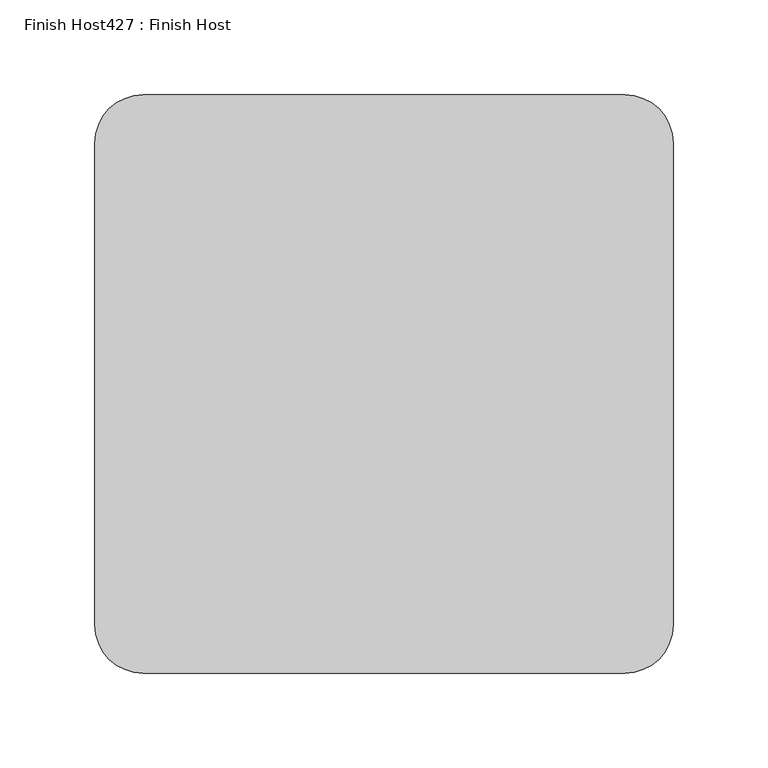
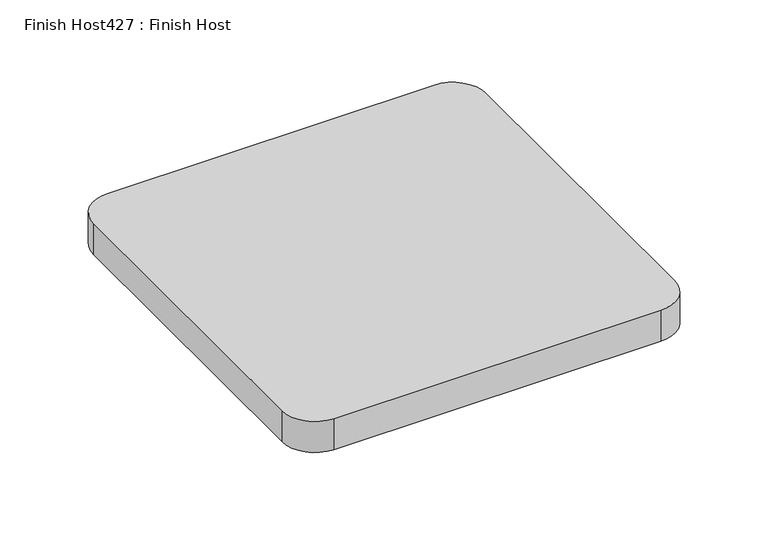
"""IFC4 building model written with IfcOpenShell, lengths in millimetres: proxy geometry, Finish Host427 : Finish Host."""

import ifcopenshell
import ifcopenshell.guid

model = None  # the IFC model being written
_history = None  # IfcOwnerHistory: only IFC2X3 demands one
_inside = {}  # id of a spatial element -> (the spatial element, [elements in it])
_under = {}  # id of a project, library or spatial element -> (it, [spatial elements below it])
_declared = {}  # id of a project -> (the project, [libraries it declares])
_typed = {}  # id of a type object -> (the type object, [elements of that type])
_made_of = {}  # id of a material, layer set ... -> (it, [elements and type objects made of it])


def new_model(schema):
    """Start an empty IFC model of exactly this schema.

    Asked for "IFC4X3", IfcOpenShell would pick the latest addendum, in which some entities
    have other attributes; the version numbers below select the first issue.
    IFC2X3 requires an IfcOwnerHistory on every rooted entity: one is made here for all.
    """
    global model, _history
    if schema == "IFC4X3":
        model = ifcopenshell.file(schema_version=(4, 3, 0, 0))
    else:
        model = ifcopenshell.file(schema=schema)
    _inside.clear()
    _under.clear()
    _declared.clear()
    _typed.clear()
    _made_of.clear()
    _history = None
    if model.schema == "IFC2X3":
        org = make("IfcOrganization", Name="unknown")
        user = make(
            "IfcPersonAndOrganization",
            ThePerson=make("IfcPerson", FamilyName="unknown"),
            TheOrganization=org,
        )
        app = make(
            "IfcApplication",
            ApplicationDeveloper=org,
            Version="unknown",
            ApplicationFullName="unknown",
            ApplicationIdentifier="unknown",
        )
        _history = make(
            "IfcOwnerHistory",
            OwningUser=user,
            OwningApplication=app,
            ChangeAction="ADDED",
            CreationDate=0,
        )
    return model


def make(cls, **values):
    """One entity of the class cls with the attributes given. An attribute that is None is left unset."""
    return model.create_entity(
        cls, **{name: value for name, value in values.items() if value is not None}
    )


def rooted(cls, **values):
    """An entity with a GlobalId (a new one), such as an element, a storey or a relation."""
    return make(cls, GlobalId=ifcopenshell.guid.new(), OwnerHistory=_history, **values)


def si_unit(unit_type, name, prefix=None):
    """IfcSIUnit, for example si_unit("LENGTHUNIT", "METRE", prefix="MILLI")."""
    return make("IfcSIUnit", UnitType=unit_type, Prefix=prefix, Name=name)


def assignment(units):
    """IfcUnitAssignment: the units of a project."""
    return None if units is None else make("IfcUnitAssignment", Units=units)


def point(xyz):
    """IfcCartesianPoint."""
    return None if xyz is None else make("IfcCartesianPoint", Coordinates=xyz)


def direction(xyz):
    """IfcDirection."""
    return None if xyz is None else make("IfcDirection", DirectionRatios=xyz)


def frame(location, z_axis=None, x_axis=None):
    """IfcAxis2Placement3D, a coordinate frame: its origin and axes. An axis left out is left unset."""
    return make(
        "IfcAxis2Placement3D",
        Location=point(location),
        Axis=direction(z_axis),
        RefDirection=direction(x_axis),
    )


def frame_2d(location, x_axis=None):
    """IfcAxis2Placement2D, a coordinate frame in the plane: its origin and x axis."""
    return make(
        "IfcAxis2Placement2D", Location=point(location), RefDirection=direction(x_axis)
    )


def origin():
    """The frame at (0, 0, 0) with its axes left unset."""
    return frame((0.0, 0.0, 0.0))


def origin_with_axes():
    """The frame at (0, 0, 0) with the z axis (0, 0, 1) and the x axis (1, 0, 0) written out."""
    return frame((0.0, 0.0, 0.0), z_axis=(0.0, 0.0, 1.0), x_axis=(1.0, 0.0, 0.0))


def place(relative_to, where):
    """IfcLocalPlacement: puts the frame where relative to a parent placement (None: the world)."""
    return make(
        "IfcLocalPlacement", PlacementRelTo=relative_to, RelativePlacement=where
    )


def context(
    kind, dimensions, precision=None, world=None, true_north=None, identifier=None
):
    """IfcGeometricRepresentationContext, for example the 3D "Model" context."""
    return make(
        "IfcGeometricRepresentationContext",
        ContextIdentifier=identifier,
        ContextType=kind,
        CoordinateSpaceDimension=dimensions,
        Precision=precision,
        WorldCoordinateSystem=world,
        TrueNorth=true_north,
    )


def project(units=None, contexts=None):
    """IfcProject with its units and contexts."""
    return rooted(
        "IfcProject",
        Name="project",
        RepresentationContexts=contexts,
        UnitsInContext=assignment(units),
    )


def spatial(cls, under=None, at=None, **own):
    """A site, building, storey or space (cls), placed at a placement, below another one or the project."""
    s = rooted(cls, ObjectPlacement=at, **own)
    if under is not None:
        _under.setdefault(under.id(), (under, []))[1].append(s)
    return s


def polyline(points):
    """IfcPolyline through the points."""
    return make("IfcPolyline", Points=[point(p) for p in points])


def circle_curve(where, radius):
    """IfcCircle in the frame where."""
    return make("IfcCircle", Position=where, Radius=radius)


def trimmed(basis, trim1, trim2, sense, master):
    """IfcTrimmedCurve: the piece of a basis curve between two trims."""
    return make(
        "IfcTrimmedCurve",
        BasisCurve=basis,
        Trim1=trim1,
        Trim2=trim2,
        SenseAgreement=sense,
        MasterRepresentation=master,
    )


def segment(curve, same_sense, transition):
    """IfcCompositeCurveSegment."""
    return make(
        "IfcCompositeCurveSegment",
        Transition=transition,
        SameSense=same_sense,
        ParentCurve=curve,
    )


def composite_curve(segments, self_intersect=None):
    """IfcCompositeCurve: segments joined end to end."""
    return make("IfcCompositeCurve", Segments=segments, SelfIntersect=self_intersect)


def outline(outer, holes=None, kind="AREA"):
    """IfcArbitraryClosedProfileDef: a profile drawn as a closed curve; with holes, ...WithVoids."""
    if holes is None:
        return make("IfcArbitraryClosedProfileDef", ProfileType=kind, OuterCurve=outer)
    return make(
        "IfcArbitraryProfileDefWithVoids",
        ProfileType=kind,
        OuterCurve=outer,
        InnerCurves=holes,
    )


def extrude(swept, where, along, depth):
    """IfcExtrudedAreaSolid: the profile swept, set in the frame where, extruded along a direction by depth."""
    return make(
        "IfcExtrudedAreaSolid",
        SweptArea=swept,
        Position=where,
        ExtrudedDirection=direction(along),
        Depth=depth,
    )


def shape(context_of_items, identifier, shape_type, items):
    """IfcShapeRepresentation: the items that make up one representation, for example the "Body"."""
    return make(
        "IfcShapeRepresentation",
        ContextOfItems=context_of_items,
        RepresentationIdentifier=identifier,
        RepresentationType=shape_type,
        Items=items,
    )


def source(mapping_origin, context_of_items, identifier, shape_type, items):
    """IfcRepresentationMap: a shape defined once, which mapped items show again and again."""
    return make(
        "IfcRepresentationMap",
        MappingOrigin=mapping_origin,
        MappedRepresentation=shape(context_of_items, identifier, shape_type, items),
    )


def transform(
    local_origin,
    x_axis=None,
    y_axis=None,
    z_axis=None,
    scale=None,
    scale2=None,
    scale3=None,
    uniform=True,
):
    """IfcCartesianTransformationOperator3D, or its non-uniform kind. x_axis, y_axis, z_axis: its Axis1, 2, 3."""
    if uniform:
        return make(
            "IfcCartesianTransformationOperator3D",
            Axis1=direction(x_axis),
            Axis2=direction(y_axis),
            LocalOrigin=point(local_origin),
            Scale=scale,
            Axis3=direction(z_axis),
        )
    return make(
        "IfcCartesianTransformationOperator3DnonUniform",
        Axis1=direction(x_axis),
        Axis2=direction(y_axis),
        LocalOrigin=point(local_origin),
        Scale=scale,
        Axis3=direction(z_axis),
        Scale2=scale2,
        Scale3=scale3,
    )


def mapped(mapping_source, mapping_target):
    """IfcMappedItem: shows the shape of a source again, moved by a transform."""
    return make(
        "IfcMappedItem", MappingSource=mapping_source, MappingTarget=mapping_target
    )


def made_of(thing, what):
    """Note that an element or type object is made of a material, layer set ...; save() writes the relation."""
    if what is not None:
        _made_of.setdefault(what.id(), (what, []))[1].append(thing)
    return thing


def element(
    cls,
    number,
    at=None,
    inside=None,
    cuts=None,
    type_object=None,
    material=None,
    context=None,
    identifier="Body",
    shape_type=None,
    held_by="IfcProductDefinitionShape",
    body=None,
    shapes=None,
    **own,
):
    """One element of the class cls, such as IfcWall. Its Tag is "e" and its number.

    at: its placement. inside: the storey or other place that contains it. cuts: it is an
    opening in that element (IfcRelVoidsElement). A single representation is given by context,
    identifier, shape_type and body (its items); several are given by shapes. held_by: the class
    of the entity that holds the representations. save() writes the other relations.
    """
    e = rooted(cls, Tag="e%d" % number, ObjectPlacement=at, **own)
    if body is not None:
        shapes = [shape(context, identifier, shape_type, body)]
    if shapes is not None:
        e.Representation = make(held_by, Representations=shapes)
    if inside is not None:
        _inside.setdefault(inside.id(), (inside, []))[1].append(e)
    if cuts is not None:
        rooted(
            "IfcRelVoidsElement", RelatingBuildingElement=cuts, RelatedOpeningElement=e
        )
    if type_object is not None:
        _typed.setdefault(type_object.id(), (type_object, []))[1].append(e)
    return made_of(e, material)


def aggregate(whole, parts):
    """IfcRelAggregates: a whole, such as a stair, and the parts it consists of."""
    return rooted("IfcRelAggregates", RelatingObject=whole, RelatedObjects=parts)


def save(model, path):
    """Write the relations noted so far, then the file.

    IfcRelAggregates (storeys below a building ...), IfcRelContainedInSpatialStructure (elements
    in a storey), IfcRelDefinesByType, IfcRelAssociatesMaterial and IfcRelDeclares: one each for
    every whole, place, type object, material and project.
    """
    for whole, parts in _under.values():
        aggregate(whole, parts)
    for where, things in _inside.values():
        rooted(
            "IfcRelContainedInSpatialStructure",
            RelatedElements=things,
            RelatingStructure=where,
        )
    for kind, things in _typed.values():
        rooted("IfcRelDefinesByType", RelatedObjects=things, RelatingType=kind)
    for what, things in _made_of.values():
        rooted("IfcRelAssociatesMaterial", RelatedObjects=things, RelatingMaterial=what)
    for by, libraries in _declared.values():
        rooted("IfcRelDeclares", RelatingContext=by, RelatedDefinitions=libraries)
    model.write(path)


def finish_host427_finish_host_3da12115(model_context):
    return source(origin(), model_context, "Body", "SweptSolid", [
        extrude(outline(composite_curve([segment(polyline([(-10878.637433, 9056.8675603), (-10878.637433, 9310.8675603)]), True, "CONTINUOUS"), segment(trimmed(circle_curve(frame_2d((-10853.237433, 9310.8675603)), 25.4), [point((-10878.637433, 9310.8675603))], [point((-10853.237433, 9336.2675603))], False, "CARTESIAN"), True, "CONTINUOUS"), segment(polyline([(-10853.237433, 9336.2675603), (-10599.237433, 9336.2675603)]), True, "CONTINUOUS"), segment(trimmed(circle_curve(frame_2d((-10599.237433, 9310.8675603)), 25.4), [point((-10599.237433, 9336.2675603))], [point((-10573.837433, 9310.8675603))], False, "CARTESIAN"), True, "CONTINUOUS"), segment(polyline([(-10573.837433, 9310.8675603), (-10573.837433, 9056.8675603)]), True, "CONTINUOUS"), segment(trimmed(circle_curve(frame_2d((-10599.237433, 9056.8675603)), 25.4), [point((-10573.837433, 9056.8675603))], [point((-10599.237433, 9031.4675603))], False, "CARTESIAN"), True, "CONTINUOUS"), segment(polyline([(-10599.237433, 9031.4675603), (-10853.237433, 9031.4675603)]), True, "CONTINUOUS"), segment(trimmed(circle_curve(frame_2d((-10853.237433, 9056.8675603)), 25.4), [point((-10853.237433, 9031.4675603))], [point((-10878.637433, 9056.8675603))], False, "CARTESIAN"), True, "CONTINUOUS")], self_intersect=False)), origin_with_axes(), (0.0, 0.0, 1.0), 25.4),
    ])


if __name__ == "__main__":
    model = new_model("IFC4")
    model_context = context("Model", 3, world=origin())
    ifc_project = project(units=[si_unit("LENGTHUNIT", "METRE", prefix="MILLI")], contexts=[model_context])
    site = spatial("IfcSite", under=ifc_project)
    building = spatial("IfcBuilding", under=site)
    placement = place(None, origin())
    finish_host427_finish_host_shape = finish_host427_finish_host_3da12115(model_context)
    element("IfcBuildingElementProxy", 1, Name="Finish Host427 : Finish Host", ObjectType="Finish Host427 : Finish Host", at=placement, inside=building, context=model_context, shape_type="MappedRepresentation", body=[
        mapped(finish_host427_finish_host_shape, transform((0.0, 0.0, 0.0), x_axis=(1.0, 0.0, 0.0), y_axis=(0.0, 1.0, 0.0), z_axis=(0.0, 0.0, 1.0))),
    ])
    save(model, "model.ifc")

# Revit data of these elements
# Type "Finish Host427 : Finish Host"
#   Panel Material = Paint - Teknion - Accent - Terracotta
# Element 1 (IfcBuildingElementProxy, "Finish Host427 : Finish Host")
#   Materials on its faces: "Paint - Teknion - Accent - Terracotta"
# Materials
#   "Paint - Teknion - Accent - Terracotta": class "Paint", colour RGB 154 112 74, transparency 0, Manufacturer = "Teknion", URL = "http://www.teknion.com/", Description = "Terracotta", Cost = 0
